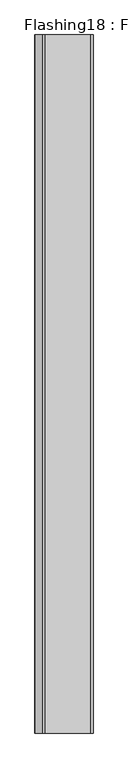
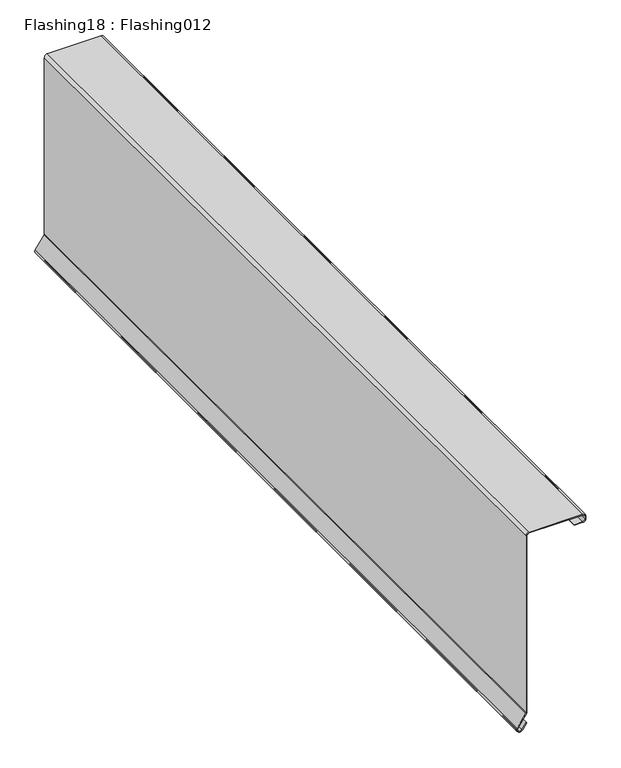
"""IFC4 building model written with IfcOpenShell, lengths in millimetres: proxy geometry, Flashing18 : Flashing012."""

from ifc_helpers import new_model, si_unit, point, frame, frame_2d, origin, place, context, project, spatial, polyline, circle_curve, trimmed, segment, composite_curve, outline, extrude, source, transform, mapped, element, save


def flashing18_flashing012_affd795f(model_context):
    return source(origin(), model_context, "Body", "SweptSolid", [
        extrude(outline(composite_curve([segment(trimmed(circle_curve(frame_2d((42111.5532705, -2482.9530802)), 5.08), [point((42108.6312101, -2478.7976063))], [point((42107.4417652, -2485.9366895))], True, "CARTESIAN"), True, "CONTINUOUS"), segment(polyline([(42107.4417652, -2485.9366895), (42108.7344443, -2487.718041)]), True, "CONTINUOUS"), segment(trimmed(circle_curve(frame_2d((42112.8459496, -2484.7344317)), 5.08), [point((42108.7344443, -2487.718041))], [point((42115.753039, -2488.9003927))], True, "CARTESIAN"), True, "CONTINUOUS"), segment(polyline([(42115.753039, -2488.9003927), (42146.0058896, -2467.7893589)]), True, "CONTINUOUS"), segment(trimmed(circle_curve(frame_2d((42148.9129791, -2471.9553199)), 5.08), [point((42146.0058896, -2467.7893589))], [point((42148.9129791, -2466.8753199))], False, "CARTESIAN"), True, "CONTINUOUS"), segment(polyline([(42148.9129791, -2466.8753199), (42596.1419896, -2466.8753199)]), True, "CONTINUOUS"), segment(trimmed(circle_curve(frame_2d((42596.1419896, -2461.7953199)), 5.08), [point((42596.1419896, -2466.8753199))], [point((42601.2219896, -2461.7953199))], True, "CARTESIAN"), True, "CONTINUOUS"), segment(polyline([(42601.2219896, -2461.7953199), (42601.2219896, -2332.4553199)]), True, "CONTINUOUS"), segment(trimmed(circle_curve(frame_2d((42596.1419896, -2332.4553199)), 5.08), [point((42601.2219896, -2332.4553199))], [point((42596.1419896, -2327.3753199))], True, "CARTESIAN"), True, "CONTINUOUS"), segment(polyline([(42596.1419896, -2327.3753199), (42589.7355833, -2327.3753199)]), True, "CONTINUOUS"), segment(trimmed(circle_curve(frame_2d((42589.7355833, -2332.4553199)), 5.08), [point((42589.7355833, -2327.3753199))], [point((42584.6555833, -2332.4553199))], True, "CARTESIAN"), True, "CONTINUOUS"), segment(polyline([(42584.6555833, -2332.4553199), (42584.6555833, -2353.7517847), (42582.6555833, -2353.7517847), (42582.6555833, -2332.4553199)]), True, "CONTINUOUS"), segment(trimmed(circle_curve(frame_2d((42589.7355833, -2332.4553199)), 7.08), [point((42582.6555833, -2332.4553199))], [point((42589.7355833, -2325.3753199))], False, "CARTESIAN"), True, "CONTINUOUS"), segment(polyline([(42589.7355833, -2325.3753199), (42596.1419896, -2325.3753199)]), True, "CONTINUOUS"), segment(trimmed(circle_curve(frame_2d((42596.1419896, -2332.4553199)), 7.08), [point((42596.1419896, -2325.3753199))], [point((42603.2219896, -2332.4553199))], False, "CARTESIAN"), True, "CONTINUOUS"), segment(polyline([(42603.2219896, -2332.4553199), (42603.2219896, -2461.7953199)]), True, "CONTINUOUS"), segment(trimmed(circle_curve(frame_2d((42596.1419896, -2461.7953199)), 7.08), [point((42603.2219896, -2461.7953199))], [point((42596.1419896, -2468.8753199))], False, "CARTESIAN"), True, "CONTINUOUS"), segment(polyline([(42596.1419896, -2468.8753199), (42148.9129791, -2468.8753199)]), True, "CONTINUOUS"), segment(trimmed(circle_curve(frame_2d((42148.9129791, -2471.9553199)), 3.08), [point((42148.9129791, -2468.8753199))], [point((42147.150413, -2469.429501))], True, "CARTESIAN"), True, "CONTINUOUS"), segment(polyline([(42147.150413, -2469.429501), (42116.8975624, -2490.5405348)]), True, "CONTINUOUS"), segment(trimmed(circle_curve(frame_2d((42112.8459496, -2484.7344317)), 7.08), [point((42116.8975624, -2490.5405348))], [point((42107.1157415, -2488.8926904))], False, "CARTESIAN"), True, "CONTINUOUS"), segment(polyline([(42107.1157415, -2488.8926904), (42105.8230624, -2487.1113389)]), True, "CONTINUOUS"), segment(trimmed(circle_curve(frame_2d((42111.5532705, -2482.9530802)), 7.08), [point((42105.8230624, -2487.1113389))], [point((42107.4807927, -2477.161593))], False, "CARTESIAN"), True, "CONTINUOUS"), segment(polyline([(42107.4807927, -2477.161593), (42122.0676658, -2466.9043456), (42123.2180833, -2468.5403589), (42108.6312101, -2478.7976063)]), True, "CONTINUOUS")], self_intersect=False)), frame((0.0, -1052.8906574, 0.0), z_axis=(0.0, 1.0, 0.0), x_axis=(0.0, 0.0, 1.0)), (0.0, 0.0, 1.0), 2000.0),
    ])


if __name__ == "__main__":
    model = new_model("IFC4")
    model_context = context("Model", 3, world=origin())
    ifc_project = project(units=[si_unit("LENGTHUNIT", "METRE", prefix="MILLI")], contexts=[model_context])
    site = spatial("IfcSite", under=ifc_project)
    building = spatial("IfcBuilding", under=site)
    placement = place(None, origin())
    flashing18_flashing012_shape = flashing18_flashing012_affd795f(model_context)
    element("IfcBuildingElementProxy", 1, Name="Flashing18 : Flashing012", ObjectType="Flashing18 : Flashing012", at=placement, inside=building, context=model_context, shape_type="MappedRepresentation", body=[
        mapped(flashing18_flashing012_shape, transform((0.0, 0.0, 0.0), x_axis=(1.0, 0.0, 0.0), y_axis=(0.0, 1.0, 0.0), z_axis=(0.0, 0.0, 1.0))),
    ])
    save(model, "model.ifc")

# Revit data of these elements
# Type "Flashing18 : Flashing012"
#   NameOverride = "Flashing012"
# Element 1 (IfcBuildingElementProxy, "Flashing18 : Flashing012")
#   Materials on its faces: "HIGH EAVE FLASHING"
# Materials
#   "HIGH EAVE FLASHING": class "Unassigned", colour RGB 128 128 128, transparency 0, Cost = 0
